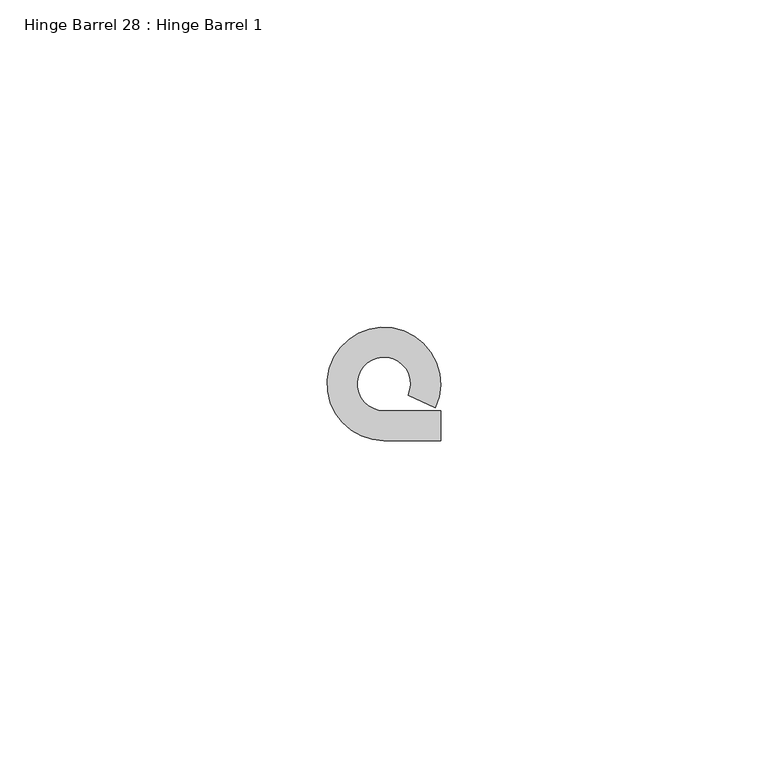
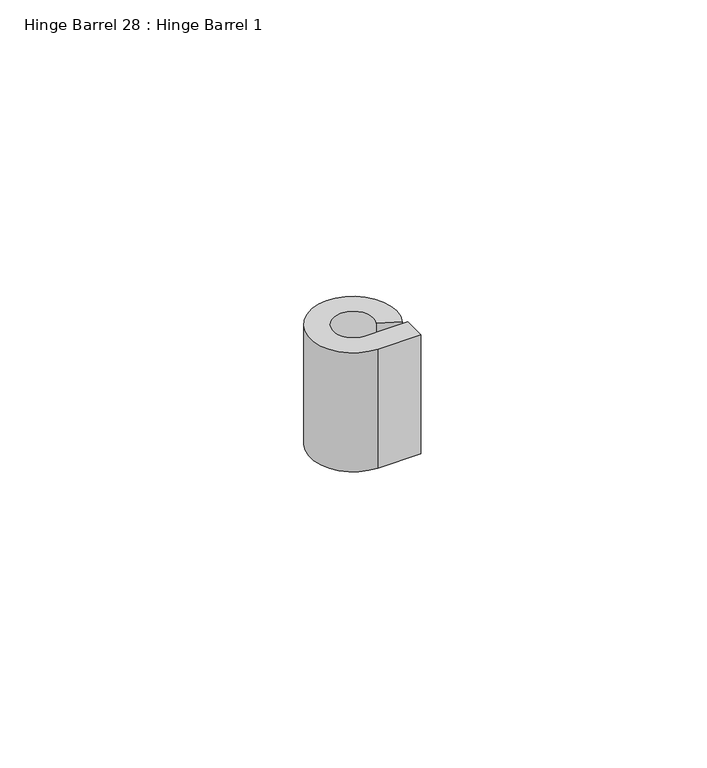
"""IFC4 building model written with IfcOpenShell, lengths in millimetres: proxy geometry, Hinge Barrel 28 : Hinge Barrel 1."""

from ifc_helpers import new_model, si_unit, point, frame, frame_2d, origin, place, context, project, spatial, polyline, circle_curve, trimmed, segment, composite_curve, outline, extrude, source, transform, mapped, element, save


def hinge_barrel_28_hinge_barrel_1_5bbaa909(model_context):
    return source(origin(), model_context, "Body", "SweptSolid", [
        extrude(outline(composite_curve([segment(polyline([(587323.2214739, -531780.6943841), (587327.7934739, -531780.6943841), (587327.7934739, -531785.2584466), (587319.1320739, -531785.2584466)]), True, "CONTINUOUS"), segment(trimmed(circle_curve(frame_2d((587319.1320739, -531776.6049841)), 8.6534625), [point((587319.1320739, -531785.2584466))], [point((587326.986084, -531780.2377433))], False, "CARTESIAN"), True, "CONTINUOUS"), segment(polyline([(587326.986084, -531780.2377433), (587322.8436736, -531778.321731)]), True, "CONTINUOUS"), segment(trimmed(circle_curve(frame_2d((587319.1320739, -531776.6049841)), 4.0894), [point((587322.8436736, -531778.321731))], [point((587319.1320739, -531780.6943841))], True, "CARTESIAN"), True, "CONTINUOUS"), segment(polyline([(587319.1320739, -531780.6943841), (587323.2214739, -531780.6943841)]), True, "CONTINUOUS")], self_intersect=False)), frame((0.0, 0.0, 1225.55), z_axis=(0.0, 0.0, 1.0), x_axis=(1.0, 0.0, 0.0)), (0.0, 0.0, 1.0), 25.4),
    ])


if __name__ == "__main__":
    model = new_model("IFC4")
    model_context = context("Model", 3, world=origin())
    ifc_project = project(units=[si_unit("LENGTHUNIT", "METRE", prefix="MILLI")], contexts=[model_context])
    site = spatial("IfcSite", under=ifc_project)
    building = spatial("IfcBuilding", under=site)
    placement = place(None, origin())
    hinge_barrel_28_hinge_barrel_1_shape = hinge_barrel_28_hinge_barrel_1_5bbaa909(model_context)
    element("IfcBuildingElementProxy", 1, Name="Hinge Barrel 28 : Hinge Barrel 1", ObjectType="Hinge Barrel 28 : Hinge Barrel 1", at=placement, inside=building, context=model_context, shape_type="MappedRepresentation", body=[
        mapped(hinge_barrel_28_hinge_barrel_1_shape, transform((0.0, 0.0, 0.0), x_axis=(1.0, 0.0, 0.0), y_axis=(0.0, 1.0, 0.0), z_axis=(0.0, 0.0, 1.0))),
    ])
    save(model, "model.ifc")

# Revit data of these elements
# Element 1 (IfcBuildingElementProxy, "Hinge Barrel 28 : Hinge Barrel 1")
#   Materials on its faces: "6\"X6\" WELD-ON STL BUTT HINGE"
# Materials
#   "6\"X6\" WELD-ON STL BUTT HINGE": class "Metal", colour RGB 189 187 185, transparency 0, Description = "Carbon steel", Cost = 0
